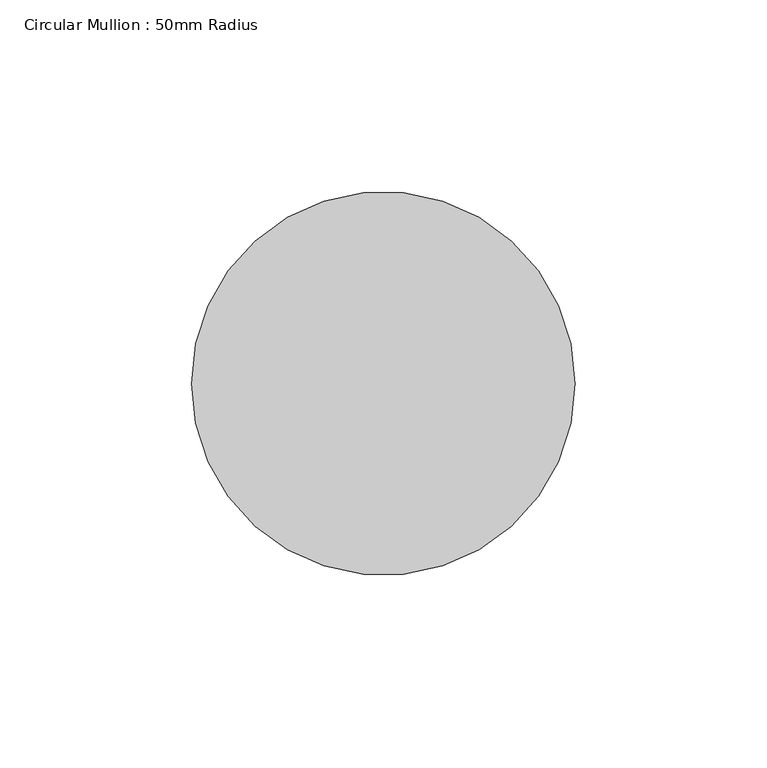
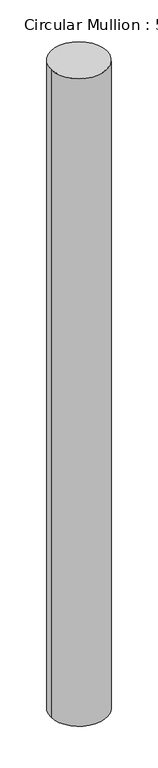
"""IFC4 building model written with IfcOpenShell, lengths in millimetres: member geometry, Circular Mullion : 50mm Radius."""

from ifc_helpers import new_model, si_unit, point, frame, origin, origin_2d, place, context, project, spatial, circle_curve, trimmed, segment, composite_curve, outline, extrude, source, transform, mapped, element, save


def circular_mullion_50mm_radius_50949ae5(model_context):
    return source(origin(), model_context, "Body", "SweptSolid", [
        extrude(outline(composite_curve([segment(trimmed(circle_curve(origin_2d(), 50.0), [point((50.0, 0.0))], [point((-50.0, 0.0))], False, "CARTESIAN"), True, "CONTINUOUS"), segment(trimmed(circle_curve(origin_2d(), 50.0), [point((-50.0, 0.0))], [point((50.0, 0.0))], False, "CARTESIAN"), True, "CONTINUOUS")], self_intersect=False)), frame((0.0, 0.0, -1227.0119158), z_axis=(0.0, 0.0, 1.0), x_axis=(1.0, 0.0, 0.0)), (0.0, 0.0, 1.0), 1227.0119158),
    ])


if __name__ == "__main__":
    model = new_model("IFC4")
    model_context = context("Model", 3, world=origin())
    ifc_project = project(units=[si_unit("LENGTHUNIT", "METRE", prefix="MILLI")], contexts=[model_context])
    site = spatial("IfcSite", under=ifc_project)
    building = spatial("IfcBuilding", under=site)
    placement = place(None, origin())
    circular_mullion_50mm_radius_shape = circular_mullion_50mm_radius_50949ae5(model_context)
    element("IfcMember", 1, ObjectType="Circular Mullion : 50mm Radius", at=placement, inside=building, context=model_context, shape_type="MappedRepresentation", body=[
        mapped(circular_mullion_50mm_radius_shape, transform((0.0, 0.0, 0.0), x_axis=(1.0, 0.0, 0.0), y_axis=(0.0, 1.0, 0.0), z_axis=(0.0, 0.0, 1.0))),
    ])
    save(model, "model.ifc")

# Revit data of these elements
# Type "Circular Mullion : 50mm Radius"
#   built-in parameter 1007350 = 0.164042 (stored number, unit not read)
# Element 1 (IfcMember, "Circular Mullion : 50mm Radius")
#   Materials on its faces: "Aluminium"
# Materials
#   "Aluminium": class "Metal", colour RGB 247 247 247, transparency 0, Description = "Aluminium 6061", Cost = 0
